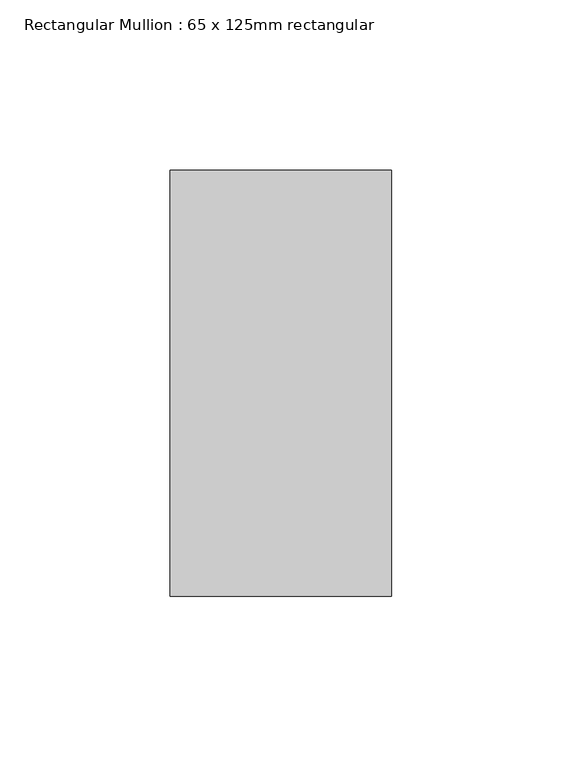
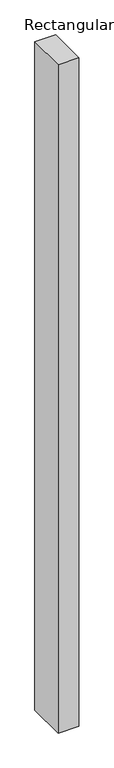
"""IFC4 building model written with IfcOpenShell, lengths in millimetres: member geometry, Rectangular Mullion : 65 x 125mm rectangular."""

from ifc_helpers import new_model, si_unit, frame, origin, place, context, project, spatial, polyline, outline, extrude, source, transform, mapped, element, save


def rectangular_mullion_65_x_125mm_rectangular_3ebb1efe(model_context):
    return source(origin(), model_context, "Body", "SweptSolid", [
        extrude(outline(polyline([(32.5, 62.5), (32.5, -62.5), (-32.5, -62.5), (-32.5, 62.5), (32.5, 62.5)])), frame((0.0, 0.0, -2200.0), z_axis=(0.0, 0.0, 1.0), x_axis=(1.0, 0.0, 0.0)), (0.0, 0.0, 1.0), 2200.0),
    ])


if __name__ == "__main__":
    model = new_model("IFC4")
    model_context = context("Model", 3, world=origin())
    ifc_project = project(units=[si_unit("LENGTHUNIT", "METRE", prefix="MILLI")], contexts=[model_context])
    site = spatial("IfcSite", under=ifc_project)
    building = spatial("IfcBuilding", under=site)
    placement = place(None, origin())
    rectangular_mullion_65_x_125mm_rectangular_shape = rectangular_mullion_65_x_125mm_rectangular_3ebb1efe(model_context)
    element("IfcMember", 1, ObjectType="Rectangular Mullion : 65 x 125mm rectangular", at=placement, inside=building, context=model_context, shape_type="MappedRepresentation", body=[
        mapped(rectangular_mullion_65_x_125mm_rectangular_shape, transform((0.0, 0.0, 0.0), x_axis=(1.0, 0.0, 0.0), y_axis=(0.0, 1.0, 0.0), z_axis=(0.0, 0.0, 1.0))),
    ])
    save(model, "model.ifc")

# Revit data of these elements
# Type "Rectangular Mullion : 65 x 125mm rectangular"
#   built-in parameter 1007304 = 0.410105 (stored number, unit not read)
#   built-in parameter 1007301 = 0.106627 (stored number, unit not read)
#   built-in parameter 1007300 = 0.106627 (stored number, unit not read)
# Element 1 (IfcMember, "Rectangular Mullion : 65 x 125mm rectangular")
#   Materials on its faces: "Aluminum"
# Materials
#   "Aluminum": class "Metal", colour RGB 244 245 246, transparency 0, Description = "Aluminum 6061", Cost = 0
